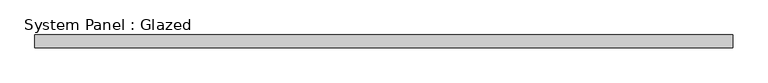
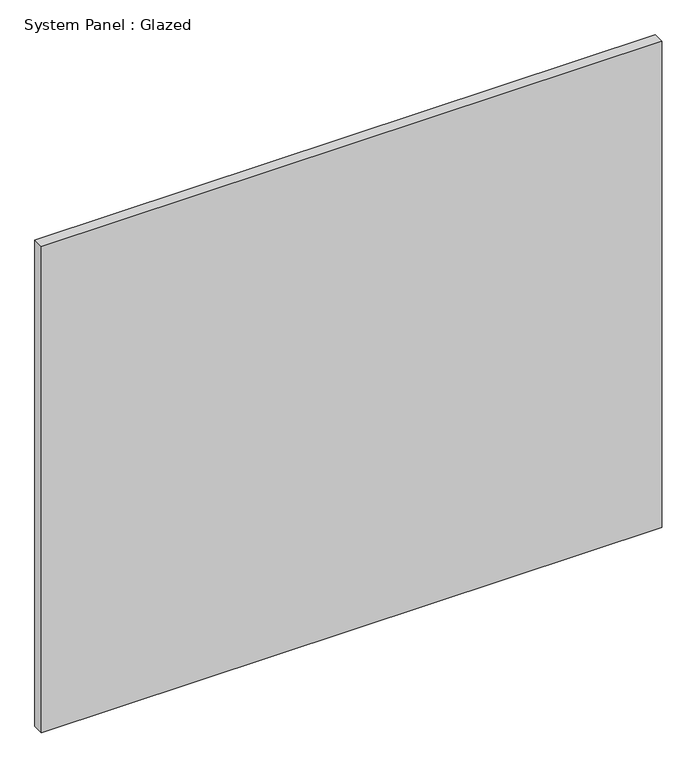
"""IFC4 building model written with IfcOpenShell, lengths in millimetres: plate geometry, System Panel : Glazed."""

import ifcopenshell
import ifcopenshell.guid

model = None  # the IFC model being written
_history = None  # IfcOwnerHistory: only IFC2X3 demands one
_inside = {}  # id of a spatial element -> (the spatial element, [elements in it])
_under = {}  # id of a project, library or spatial element -> (it, [spatial elements below it])
_declared = {}  # id of a project -> (the project, [libraries it declares])
_typed = {}  # id of a type object -> (the type object, [elements of that type])
_made_of = {}  # id of a material, layer set ... -> (it, [elements and type objects made of it])


def new_model(schema):
    """Start an empty IFC model of exactly this schema.

    Asked for "IFC4X3", IfcOpenShell would pick the latest addendum, in which some entities
    have other attributes; the version numbers below select the first issue.
    IFC2X3 requires an IfcOwnerHistory on every rooted entity: one is made here for all.
    """
    global model, _history
    if schema == "IFC4X3":
        model = ifcopenshell.file(schema_version=(4, 3, 0, 0))
    else:
        model = ifcopenshell.file(schema=schema)
    _inside.clear()
    _under.clear()
    _declared.clear()
    _typed.clear()
    _made_of.clear()
    _history = None
    if model.schema == "IFC2X3":
        org = make("IfcOrganization", Name="unknown")
        user = make(
            "IfcPersonAndOrganization",
            ThePerson=make("IfcPerson", FamilyName="unknown"),
            TheOrganization=org,
        )
        app = make(
            "IfcApplication",
            ApplicationDeveloper=org,
            Version="unknown",
            ApplicationFullName="unknown",
            ApplicationIdentifier="unknown",
        )
        _history = make(
            "IfcOwnerHistory",
            OwningUser=user,
            OwningApplication=app,
            ChangeAction="ADDED",
            CreationDate=0,
        )
    return model


def make(cls, **values):
    """One entity of the class cls with the attributes given. An attribute that is None is left unset."""
    return model.create_entity(
        cls, **{name: value for name, value in values.items() if value is not None}
    )


def rooted(cls, **values):
    """An entity with a GlobalId (a new one), such as an element, a storey or a relation."""
    return make(cls, GlobalId=ifcopenshell.guid.new(), OwnerHistory=_history, **values)


def si_unit(unit_type, name, prefix=None):
    """IfcSIUnit, for example si_unit("LENGTHUNIT", "METRE", prefix="MILLI")."""
    return make("IfcSIUnit", UnitType=unit_type, Prefix=prefix, Name=name)


def assignment(units):
    """IfcUnitAssignment: the units of a project."""
    return None if units is None else make("IfcUnitAssignment", Units=units)


def point(xyz):
    """IfcCartesianPoint."""
    return None if xyz is None else make("IfcCartesianPoint", Coordinates=xyz)


def direction(xyz):
    """IfcDirection."""
    return None if xyz is None else make("IfcDirection", DirectionRatios=xyz)


def frame(location, z_axis=None, x_axis=None):
    """IfcAxis2Placement3D, a coordinate frame: its origin and axes. An axis left out is left unset."""
    return make(
        "IfcAxis2Placement3D",
        Location=point(location),
        Axis=direction(z_axis),
        RefDirection=direction(x_axis),
    )


def origin():
    """The frame at (0, 0, 0) with its axes left unset."""
    return frame((0.0, 0.0, 0.0))


def origin_with_axes():
    """The frame at (0, 0, 0) with the z axis (0, 0, 1) and the x axis (1, 0, 0) written out."""
    return frame((0.0, 0.0, 0.0), z_axis=(0.0, 0.0, 1.0), x_axis=(1.0, 0.0, 0.0))


def place(relative_to, where):
    """IfcLocalPlacement: puts the frame where relative to a parent placement (None: the world)."""
    return make(
        "IfcLocalPlacement", PlacementRelTo=relative_to, RelativePlacement=where
    )


def context(
    kind, dimensions, precision=None, world=None, true_north=None, identifier=None
):
    """IfcGeometricRepresentationContext, for example the 3D "Model" context."""
    return make(
        "IfcGeometricRepresentationContext",
        ContextIdentifier=identifier,
        ContextType=kind,
        CoordinateSpaceDimension=dimensions,
        Precision=precision,
        WorldCoordinateSystem=world,
        TrueNorth=true_north,
    )


def project(units=None, contexts=None):
    """IfcProject with its units and contexts."""
    return rooted(
        "IfcProject",
        Name="project",
        RepresentationContexts=contexts,
        UnitsInContext=assignment(units),
    )


def spatial(cls, under=None, at=None, **own):
    """A site, building, storey or space (cls), placed at a placement, below another one or the project."""
    s = rooted(cls, ObjectPlacement=at, **own)
    if under is not None:
        _under.setdefault(under.id(), (under, []))[1].append(s)
    return s


def polyline(points):
    """IfcPolyline through the points."""
    return make("IfcPolyline", Points=[point(p) for p in points])


def outline(outer, holes=None, kind="AREA"):
    """IfcArbitraryClosedProfileDef: a profile drawn as a closed curve; with holes, ...WithVoids."""
    if holes is None:
        return make("IfcArbitraryClosedProfileDef", ProfileType=kind, OuterCurve=outer)
    return make(
        "IfcArbitraryProfileDefWithVoids",
        ProfileType=kind,
        OuterCurve=outer,
        InnerCurves=holes,
    )


def extrude(swept, where, along, depth):
    """IfcExtrudedAreaSolid: the profile swept, set in the frame where, extruded along a direction by depth."""
    return make(
        "IfcExtrudedAreaSolid",
        SweptArea=swept,
        Position=where,
        ExtrudedDirection=direction(along),
        Depth=depth,
    )


def shape(context_of_items, identifier, shape_type, items):
    """IfcShapeRepresentation: the items that make up one representation, for example the "Body"."""
    return make(
        "IfcShapeRepresentation",
        ContextOfItems=context_of_items,
        RepresentationIdentifier=identifier,
        RepresentationType=shape_type,
        Items=items,
    )


def source(mapping_origin, context_of_items, identifier, shape_type, items):
    """IfcRepresentationMap: a shape defined once, which mapped items show again and again."""
    return make(
        "IfcRepresentationMap",
        MappingOrigin=mapping_origin,
        MappedRepresentation=shape(context_of_items, identifier, shape_type, items),
    )


def transform(
    local_origin,
    x_axis=None,
    y_axis=None,
    z_axis=None,
    scale=None,
    scale2=None,
    scale3=None,
    uniform=True,
):
    """IfcCartesianTransformationOperator3D, or its non-uniform kind. x_axis, y_axis, z_axis: its Axis1, 2, 3."""
    if uniform:
        return make(
            "IfcCartesianTransformationOperator3D",
            Axis1=direction(x_axis),
            Axis2=direction(y_axis),
            LocalOrigin=point(local_origin),
            Scale=scale,
            Axis3=direction(z_axis),
        )
    return make(
        "IfcCartesianTransformationOperator3DnonUniform",
        Axis1=direction(x_axis),
        Axis2=direction(y_axis),
        LocalOrigin=point(local_origin),
        Scale=scale,
        Axis3=direction(z_axis),
        Scale2=scale2,
        Scale3=scale3,
    )


def mapped(mapping_source, mapping_target):
    """IfcMappedItem: shows the shape of a source again, moved by a transform."""
    return make(
        "IfcMappedItem", MappingSource=mapping_source, MappingTarget=mapping_target
    )


def made_of(thing, what):
    """Note that an element or type object is made of a material, layer set ...; save() writes the relation."""
    if what is not None:
        _made_of.setdefault(what.id(), (what, []))[1].append(thing)
    return thing


def element(
    cls,
    number,
    at=None,
    inside=None,
    cuts=None,
    type_object=None,
    material=None,
    context=None,
    identifier="Body",
    shape_type=None,
    held_by="IfcProductDefinitionShape",
    body=None,
    shapes=None,
    **own,
):
    """One element of the class cls, such as IfcWall. Its Tag is "e" and its number.

    at: its placement. inside: the storey or other place that contains it. cuts: it is an
    opening in that element (IfcRelVoidsElement). A single representation is given by context,
    identifier, shape_type and body (its items); several are given by shapes. held_by: the class
    of the entity that holds the representations. save() writes the other relations.
    """
    e = rooted(cls, Tag="e%d" % number, ObjectPlacement=at, **own)
    if body is not None:
        shapes = [shape(context, identifier, shape_type, body)]
    if shapes is not None:
        e.Representation = make(held_by, Representations=shapes)
    if inside is not None:
        _inside.setdefault(inside.id(), (inside, []))[1].append(e)
    if cuts is not None:
        rooted(
            "IfcRelVoidsElement", RelatingBuildingElement=cuts, RelatedOpeningElement=e
        )
    if type_object is not None:
        _typed.setdefault(type_object.id(), (type_object, []))[1].append(e)
    return made_of(e, material)


def aggregate(whole, parts):
    """IfcRelAggregates: a whole, such as a stair, and the parts it consists of."""
    return rooted("IfcRelAggregates", RelatingObject=whole, RelatedObjects=parts)


def save(model, path):
    """Write the relations noted so far, then the file.

    IfcRelAggregates (storeys below a building ...), IfcRelContainedInSpatialStructure (elements
    in a storey), IfcRelDefinesByType, IfcRelAssociatesMaterial and IfcRelDeclares: one each for
    every whole, place, type object, material and project.
    """
    for whole, parts in _under.values():
        aggregate(whole, parts)
    for where, things in _inside.values():
        rooted(
            "IfcRelContainedInSpatialStructure",
            RelatedElements=things,
            RelatingStructure=where,
        )
    for kind, things in _typed.values():
        rooted("IfcRelDefinesByType", RelatedObjects=things, RelatingType=kind)
    for what, things in _made_of.values():
        rooted("IfcRelAssociatesMaterial", RelatedObjects=things, RelatingMaterial=what)
    for by, libraries in _declared.values():
        rooted("IfcRelDeclares", RelatingContext=by, RelatedDefinitions=libraries)
    model.write(path)


def system_panel_glazed_88b4eb2b(model_context):
    return source(origin(), model_context, "Body", "SweptSolid", [
        extrude(outline(polyline([(697.4416668, 19.05), (-697.4416668, 19.05), (-697.4416668, 44.45), (697.4416668, 44.45), (697.4416668, 19.05)])), origin_with_axes(), (0.0, 0.0, 1.0), 1155.7),
    ])


if __name__ == "__main__":
    model = new_model("IFC4")
    model_context = context("Model", 3, world=origin())
    ifc_project = project(units=[si_unit("LENGTHUNIT", "METRE", prefix="MILLI")], contexts=[model_context])
    site = spatial("IfcSite", under=ifc_project)
    building = spatial("IfcBuilding", under=site)
    placement = place(None, origin())
    system_panel_glazed_shape = system_panel_glazed_88b4eb2b(model_context)
    element("IfcPlate", 1, ObjectType="System Panel : Glazed", at=placement, inside=building, context=model_context, shape_type="MappedRepresentation", body=[
        mapped(system_panel_glazed_shape, transform((0.0, 0.0, 0.0), x_axis=(1.0, 0.0, 0.0), y_axis=(0.0, 1.0, 0.0), z_axis=(0.0, 0.0, 1.0))),
    ])
    save(model, "model.ifc")

# Revit data of these elements
# Type "System Panel : Glazed"
#   Construction Type Id = "GSP4R"
#   Analytic Construction = "1/8 in Pilkington single glazing"
#   Visual Light Transmittance = 0.9
#   Solar Heat Gain Coefficient = 0.86
#   Heat Transfer Coefficient (U) = 1.18115 BTU/(h·ft²·°F)
#   Define Thermal Properties by = 1
# Element 1 (IfcPlate, "System Panel : Glazed")
#   Materials on its faces: "Glass"
# Materials
#   "Glass": class "Glass", colour RGB 0 128 192, transparency 0.75, Description = "Soda Lime Glass", Cost = 0
